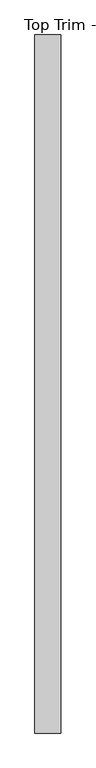
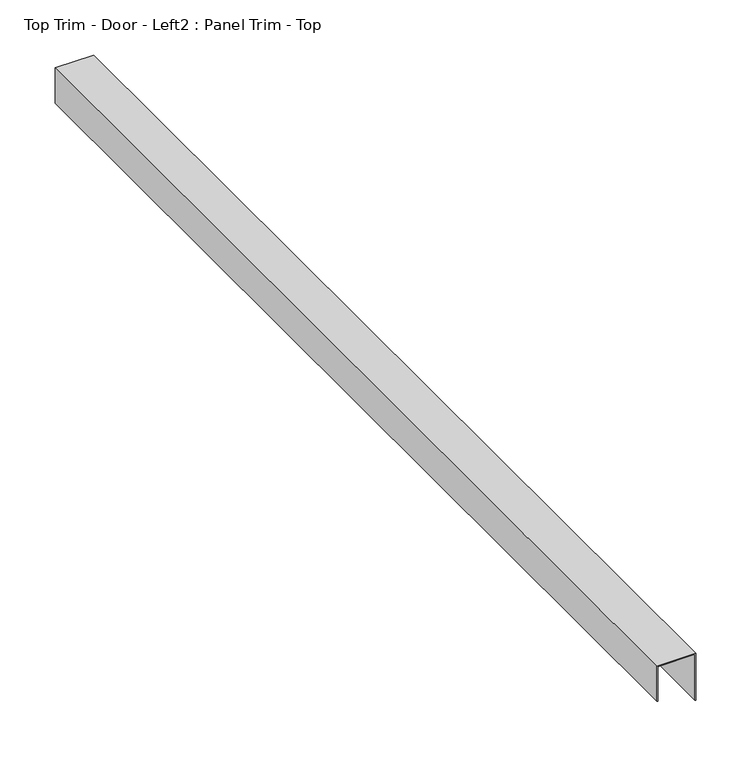
"""IFC4 building model written with IfcOpenShell, lengths in millimetres: proxy geometry, Top Trim - Door - Left2 : Panel Trim - Top."""

import ifcopenshell
import ifcopenshell.guid

model = None  # the IFC model being written
_history = None  # IfcOwnerHistory: only IFC2X3 demands one
_inside = {}  # id of a spatial element -> (the spatial element, [elements in it])
_under = {}  # id of a project, library or spatial element -> (it, [spatial elements below it])
_declared = {}  # id of a project -> (the project, [libraries it declares])
_typed = {}  # id of a type object -> (the type object, [elements of that type])
_made_of = {}  # id of a material, layer set ... -> (it, [elements and type objects made of it])


def new_model(schema):
    """Start an empty IFC model of exactly this schema.

    Asked for "IFC4X3", IfcOpenShell would pick the latest addendum, in which some entities
    have other attributes; the version numbers below select the first issue.
    IFC2X3 requires an IfcOwnerHistory on every rooted entity: one is made here for all.
    """
    global model, _history
    if schema == "IFC4X3":
        model = ifcopenshell.file(schema_version=(4, 3, 0, 0))
    else:
        model = ifcopenshell.file(schema=schema)
    _inside.clear()
    _under.clear()
    _declared.clear()
    _typed.clear()
    _made_of.clear()
    _history = None
    if model.schema == "IFC2X3":
        org = make("IfcOrganization", Name="unknown")
        user = make(
            "IfcPersonAndOrganization",
            ThePerson=make("IfcPerson", FamilyName="unknown"),
            TheOrganization=org,
        )
        app = make(
            "IfcApplication",
            ApplicationDeveloper=org,
            Version="unknown",
            ApplicationFullName="unknown",
            ApplicationIdentifier="unknown",
        )
        _history = make(
            "IfcOwnerHistory",
            OwningUser=user,
            OwningApplication=app,
            ChangeAction="ADDED",
            CreationDate=0,
        )
    return model


def make(cls, **values):
    """One entity of the class cls with the attributes given. An attribute that is None is left unset."""
    return model.create_entity(
        cls, **{name: value for name, value in values.items() if value is not None}
    )


def rooted(cls, **values):
    """An entity with a GlobalId (a new one), such as an element, a storey or a relation."""
    return make(cls, GlobalId=ifcopenshell.guid.new(), OwnerHistory=_history, **values)


def si_unit(unit_type, name, prefix=None):
    """IfcSIUnit, for example si_unit("LENGTHUNIT", "METRE", prefix="MILLI")."""
    return make("IfcSIUnit", UnitType=unit_type, Prefix=prefix, Name=name)


def assignment(units):
    """IfcUnitAssignment: the units of a project."""
    return None if units is None else make("IfcUnitAssignment", Units=units)


def point(xyz):
    """IfcCartesianPoint."""
    return None if xyz is None else make("IfcCartesianPoint", Coordinates=xyz)


def direction(xyz):
    """IfcDirection."""
    return None if xyz is None else make("IfcDirection", DirectionRatios=xyz)


def frame(location, z_axis=None, x_axis=None):
    """IfcAxis2Placement3D, a coordinate frame: its origin and axes. An axis left out is left unset."""
    return make(
        "IfcAxis2Placement3D",
        Location=point(location),
        Axis=direction(z_axis),
        RefDirection=direction(x_axis),
    )


def origin():
    """The frame at (0, 0, 0) with its axes left unset."""
    return frame((0.0, 0.0, 0.0))


def place(relative_to, where):
    """IfcLocalPlacement: puts the frame where relative to a parent placement (None: the world)."""
    return make(
        "IfcLocalPlacement", PlacementRelTo=relative_to, RelativePlacement=where
    )


def context(
    kind, dimensions, precision=None, world=None, true_north=None, identifier=None
):
    """IfcGeometricRepresentationContext, for example the 3D "Model" context."""
    return make(
        "IfcGeometricRepresentationContext",
        ContextIdentifier=identifier,
        ContextType=kind,
        CoordinateSpaceDimension=dimensions,
        Precision=precision,
        WorldCoordinateSystem=world,
        TrueNorth=true_north,
    )


def project(units=None, contexts=None):
    """IfcProject with its units and contexts."""
    return rooted(
        "IfcProject",
        Name="project",
        RepresentationContexts=contexts,
        UnitsInContext=assignment(units),
    )


def spatial(cls, under=None, at=None, **own):
    """A site, building, storey or space (cls), placed at a placement, below another one or the project."""
    s = rooted(cls, ObjectPlacement=at, **own)
    if under is not None:
        _under.setdefault(under.id(), (under, []))[1].append(s)
    return s


def polyline(points):
    """IfcPolyline through the points."""
    return make("IfcPolyline", Points=[point(p) for p in points])


def outline(outer, holes=None, kind="AREA"):
    """IfcArbitraryClosedProfileDef: a profile drawn as a closed curve; with holes, ...WithVoids."""
    if holes is None:
        return make("IfcArbitraryClosedProfileDef", ProfileType=kind, OuterCurve=outer)
    return make(
        "IfcArbitraryProfileDefWithVoids",
        ProfileType=kind,
        OuterCurve=outer,
        InnerCurves=holes,
    )


def extrude(swept, where, along, depth):
    """IfcExtrudedAreaSolid: the profile swept, set in the frame where, extruded along a direction by depth."""
    return make(
        "IfcExtrudedAreaSolid",
        SweptArea=swept,
        Position=where,
        ExtrudedDirection=direction(along),
        Depth=depth,
    )


def shape(context_of_items, identifier, shape_type, items):
    """IfcShapeRepresentation: the items that make up one representation, for example the "Body"."""
    return make(
        "IfcShapeRepresentation",
        ContextOfItems=context_of_items,
        RepresentationIdentifier=identifier,
        RepresentationType=shape_type,
        Items=items,
    )


def source(mapping_origin, context_of_items, identifier, shape_type, items):
    """IfcRepresentationMap: a shape defined once, which mapped items show again and again."""
    return make(
        "IfcRepresentationMap",
        MappingOrigin=mapping_origin,
        MappedRepresentation=shape(context_of_items, identifier, shape_type, items),
    )


def transform(
    local_origin,
    x_axis=None,
    y_axis=None,
    z_axis=None,
    scale=None,
    scale2=None,
    scale3=None,
    uniform=True,
):
    """IfcCartesianTransformationOperator3D, or its non-uniform kind. x_axis, y_axis, z_axis: its Axis1, 2, 3."""
    if uniform:
        return make(
            "IfcCartesianTransformationOperator3D",
            Axis1=direction(x_axis),
            Axis2=direction(y_axis),
            LocalOrigin=point(local_origin),
            Scale=scale,
            Axis3=direction(z_axis),
        )
    return make(
        "IfcCartesianTransformationOperator3DnonUniform",
        Axis1=direction(x_axis),
        Axis2=direction(y_axis),
        LocalOrigin=point(local_origin),
        Scale=scale,
        Axis3=direction(z_axis),
        Scale2=scale2,
        Scale3=scale3,
    )


def mapped(mapping_source, mapping_target):
    """IfcMappedItem: shows the shape of a source again, moved by a transform."""
    return make(
        "IfcMappedItem", MappingSource=mapping_source, MappingTarget=mapping_target
    )


def made_of(thing, what):
    """Note that an element or type object is made of a material, layer set ...; save() writes the relation."""
    if what is not None:
        _made_of.setdefault(what.id(), (what, []))[1].append(thing)
    return thing


def element(
    cls,
    number,
    at=None,
    inside=None,
    cuts=None,
    type_object=None,
    material=None,
    context=None,
    identifier="Body",
    shape_type=None,
    held_by="IfcProductDefinitionShape",
    body=None,
    shapes=None,
    **own,
):
    """One element of the class cls, such as IfcWall. Its Tag is "e" and its number.

    at: its placement. inside: the storey or other place that contains it. cuts: it is an
    opening in that element (IfcRelVoidsElement). A single representation is given by context,
    identifier, shape_type and body (its items); several are given by shapes. held_by: the class
    of the entity that holds the representations. save() writes the other relations.
    """
    e = rooted(cls, Tag="e%d" % number, ObjectPlacement=at, **own)
    if body is not None:
        shapes = [shape(context, identifier, shape_type, body)]
    if shapes is not None:
        e.Representation = make(held_by, Representations=shapes)
    if inside is not None:
        _inside.setdefault(inside.id(), (inside, []))[1].append(e)
    if cuts is not None:
        rooted(
            "IfcRelVoidsElement", RelatingBuildingElement=cuts, RelatedOpeningElement=e
        )
    if type_object is not None:
        _typed.setdefault(type_object.id(), (type_object, []))[1].append(e)
    return made_of(e, material)


def aggregate(whole, parts):
    """IfcRelAggregates: a whole, such as a stair, and the parts it consists of."""
    return rooted("IfcRelAggregates", RelatingObject=whole, RelatedObjects=parts)


def save(model, path):
    """Write the relations noted so far, then the file.

    IfcRelAggregates (storeys below a building ...), IfcRelContainedInSpatialStructure (elements
    in a storey), IfcRelDefinesByType, IfcRelAssociatesMaterial and IfcRelDeclares: one each for
    every whole, place, type object, material and project.
    """
    for whole, parts in _under.values():
        aggregate(whole, parts)
    for where, things in _inside.values():
        rooted(
            "IfcRelContainedInSpatialStructure",
            RelatedElements=things,
            RelatingStructure=where,
        )
    for kind, things in _typed.values():
        rooted("IfcRelDefinesByType", RelatedObjects=things, RelatingType=kind)
    for what, things in _made_of.values():
        rooted("IfcRelAssociatesMaterial", RelatedObjects=things, RelatingMaterial=what)
    for by, libraries in _declared.values():
        rooted("IfcRelDeclares", RelatingContext=by, RelatedDefinitions=libraries)
    model.write(path)


def top_trim_door_left2_panel_trim_top_4d2a0b62(model_context):
    return source(origin(), model_context, "Body", "SweptSolid", [
        extrude(outline(polyline([(2438.4, 587327.0060739), (2438.4, 587365.8934739), (2387.6, 587365.8934739), (2387.6, 587366.6808739), (2439.19375, 587366.6808739), (2439.19375, 587326.2186739), (2400.3, 587326.2186739), (2400.3, 587327.0060739), (2438.4, 587327.0060739)])), frame((0.0, -532877.4663841, 0.0), z_axis=(0.0, 1.0, 0.0), x_axis=(0.0, 0.0, 1.0)), (0.0, 0.0, 1.0), 1092.2),
    ])


if __name__ == "__main__":
    model = new_model("IFC4")
    model_context = context("Model", 3, world=origin())
    ifc_project = project(units=[si_unit("LENGTHUNIT", "METRE", prefix="MILLI")], contexts=[model_context])
    site = spatial("IfcSite", under=ifc_project)
    building = spatial("IfcBuilding", under=site)
    placement = place(None, origin())
    top_trim_door_left2_panel_trim_top_shape = top_trim_door_left2_panel_trim_top_4d2a0b62(model_context)
    element("IfcBuildingElementProxy", 1, Name="Top Trim - Door - Left2 : Panel Trim - Top", ObjectType="Top Trim - Door - Left2 : Panel Trim - Top", at=placement, inside=building, context=model_context, shape_type="MappedRepresentation", body=[
        mapped(top_trim_door_left2_panel_trim_top_shape, transform((0.0, 0.0, 0.0), x_axis=(1.0, 0.0, 0.0), y_axis=(0.0, 1.0, 0.0), z_axis=(0.0, 0.0, 1.0))),
    ])
    save(model, "model.ifc")

# Revit data of these elements
# Element 1 (IfcBuildingElementProxy, "Top Trim - Door - Left2 : Panel Trim - Top")
#   Materials on its faces: "EDGE TRIM BY MTL PANEL MFR."
# Materials
#   "EDGE TRIM BY MTL PANEL MFR.": class "Generic", colour RGB 239 242 240, transparency 0, Cost = 0
